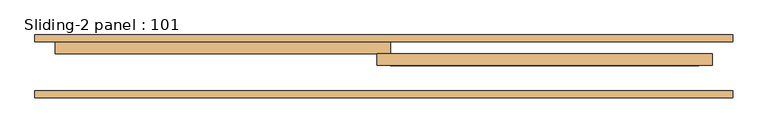
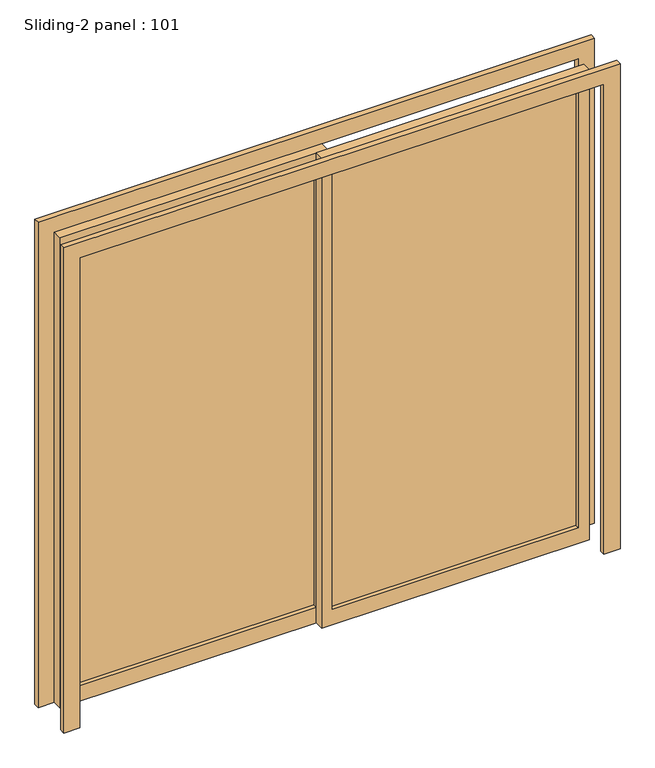
"""IFC4 building model written with IfcOpenShell, lengths in millimetres: door geometry, Sliding-2 panel : 101."""

from ifc_helpers import new_model, si_unit, frame, origin, place, context, project, spatial, polyline, outline, extrude, source, transform, mapped, element, save


def sliding_2_panel_101_c3ea5440(model_context):
    return source(origin(), model_context, "Body", "SweptSolid", [
        extrude(outline(polyline([(25.4, 155.575), (1181.1, 155.575), (1181.1, 149.225), (25.4, 149.225), (25.4, 155.575)])), frame((0.0, 0.0, 76.2), z_axis=(0.0, 0.0, 1.0), x_axis=(1.0, 0.0, 0.0)), (0.0, 0.0, 1.0), 2184.4),
        extrude(outline(polyline([(2336.8, -25.4), (0.0, -25.4), (0.0, 1231.9), (2336.8, 1231.9), (2336.8, -25.4)]), holes=[polyline([(2260.6, 25.4), (2260.6, 1181.1), (76.2, 1181.1), (76.2, 25.4), (2260.6, 25.4)])]), frame((0.0, 130.175, 0.0), z_axis=(0.0, 1.0, 0.0), x_axis=(0.0, 0.0, 1.0)), (0.0, 0.0, 1.0), 44.45),
        extrude(outline(polyline([(-1181.1, 200.025), (-25.4, 200.025), (-25.4, 193.675), (-1181.1, 193.675), (-1181.1, 200.025)])), frame((0.0, 0.0, 76.2), z_axis=(0.0, 0.0, 1.0), x_axis=(1.0, 0.0, 0.0)), (0.0, 0.0, 1.0), 2184.4),
        extrude(outline(polyline([(2336.8, 25.4), (2336.8, -1231.9), (0.0, -1231.9), (0.0, 25.4), (2336.8, 25.4)]), holes=[polyline([(2260.6, -25.4), (76.2, -25.4), (76.2, -1181.1), (2260.6, -1181.1), (2260.6, -25.4)])]), frame((0.0, 174.625, 0.0), z_axis=(0.0, 1.0, 0.0), x_axis=(0.0, 0.0, 1.0)), (0.0, 0.0, 1.0), 44.45),
        extrude(outline(polyline([(0.0, -1308.1), (0.0, -1231.9), (2336.8, -1231.9), (2336.8, 1231.9), (0.0, 1231.9), (0.0, 1308.1), (2413.0, 1308.1), (2413.0, -1308.1), (0.0, -1308.1)])), frame((0.0, 9.525, 0.0), z_axis=(0.0, 1.0, 0.0), x_axis=(0.0, 0.0, 1.0)), (0.0, 0.0, 1.0), 25.4),
        extrude(outline(polyline([(0.0, 1308.1), (2413.0, 1308.1), (2413.0, -1308.1), (0.0, -1308.1), (0.0, -1231.9), (2336.8, -1231.9), (2336.8, 1231.9), (0.0, 1231.9), (0.0, 1308.1)])), frame((0.0, 219.075, 0.0), z_axis=(0.0, 1.0, 0.0), x_axis=(0.0, 0.0, 1.0)), (0.0, 0.0, 1.0), 25.4),
    ])


if __name__ == "__main__":
    model = new_model("IFC4")
    model_context = context("Model", 3, world=origin())
    ifc_project = project(units=[si_unit("LENGTHUNIT", "METRE", prefix="MILLI")], contexts=[model_context])
    site = spatial("IfcSite", under=ifc_project)
    building = spatial("IfcBuilding", under=site)
    placement = place(None, origin())
    sliding_2_panel_101_shape = sliding_2_panel_101_c3ea5440(model_context)
    element("IfcDoor", 1, ObjectType="Sliding-2 panel : 101", at=placement, inside=building, context=model_context, shape_type="MappedRepresentation", body=[
        mapped(sliding_2_panel_101_shape, transform((0.0, 0.0, 0.0), x_axis=(1.0, 0.0, 0.0), y_axis=(0.0, 1.0, 0.0), z_axis=(0.0, 0.0, 1.0))),
    ])
    save(model, "model.ifc")

# Revit data of these elements
# Type "Sliding-2 panel : 101"
#   Type Mark = "101"
#   Construction Type Id = "MDOOR"
#   Assembly Code = "C1020"
#   Analytic Construction = "Metal"
#   Thickness = 0' - 1 3/4"
#   Heat Transfer Coefficient (U) = 3.7021 W/(m²·K)
#   Height = 7' - 8"
#   Rail Width = 0' - 3"
#   Stile Width = 0' - 2"
#   Trim Projection Ext = 0' - 1"
#   Trim Projection Int = 0' - 1"
#   Trim Width = 0' - 3"
#   Width = 8' - 1"
#   Door Material = 05 - Metal - Aluminum
#   Frame Material = 05 - Metal - Steel
#   Visual Light Transmittance = 0
#   Solar Heat Gain Coefficient = 0
#   Function = (empty or 0)
#   Wall Closure = (empty or 0)
# Element 1 (IfcDoor, "Sliding-2 panel : 101")
#   Materials on its faces: "05 - Metal - Aluminum", "05 - Metal - Steel", "Glass"
# Materials
#   "05 - Metal - Aluminum": class "Unassigned", colour RGB 247 247 247, transparency 0, Description = "Aluminum"
#   "05 - Metal - Steel": class "Unassigned", colour RGB 199 199 199, transparency 0, Description = "Steel"
#   "Glass": class "Unassigned", colour RGB 0 0 255, transparency 0.75
